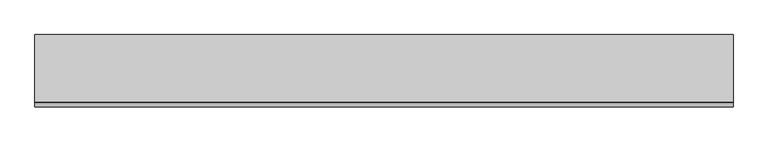
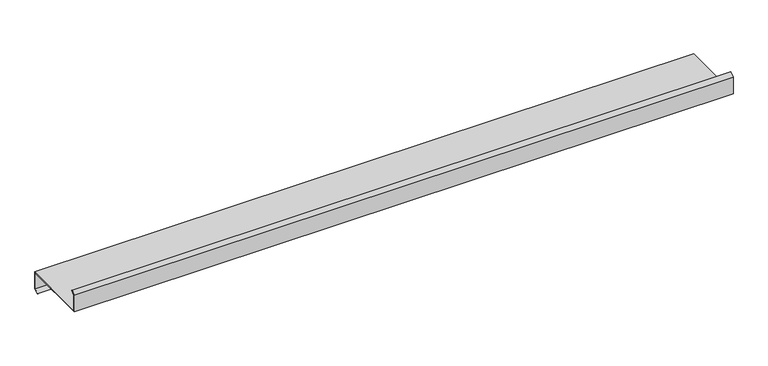
"""IFC4 building model written with IfcOpenShell, lengths in millimetres: proxy geometry, Generic Models 7:Generic Models 1:337419:Generic Models 1:337419 : Generic Models 7:Generic Models 1:337419:25 : Generic Models 7:Generic Models 1:337419:Generic Models 1:337419 : Generic Models 7:Generic Models 1:337419:301336."""

from ifc_helpers import new_model, si_unit, frame, origin, place, context, project, spatial, polyline, outline, extrude, source, transform, mapped, element, save


def generic_models_e2588900(model_context):
    return source(origin(), model_context, "Body", "SweptSolid", [
        extrude(outline(polyline([(-566667.6964303, 3711.7734375), (-566667.6964303, 3776.6625), (-566653.2894741, 3788.7513716), (-566651.3175393, 3786.7794368), (-566664.9183053, 3775.367039), (-566664.9183053, 3714.5515625), (-566413.6964303, 3714.5515625), (-566413.6964303, 3649.6625), (-566428.2895769, 3637.417396), (-566430.2615117, 3639.3893309), (-566416.4745553, 3650.957961), (-566416.4745553, 3711.7734375), (-566667.6964303, 3711.7734375)])), frame((599865.8367239, 0.0, 0.0), z_axis=(1.0, 0.0, 0.0), x_axis=(0.0, 1.0, 0.0)), (0.0, 0.0, 1.0), 2444.75),
    ])


if __name__ == "__main__":
    model = new_model("IFC4")
    model_context = context("Model", 3, world=origin())
    ifc_project = project(units=[si_unit("LENGTHUNIT", "METRE", prefix="MILLI")], contexts=[model_context])
    site = spatial("IfcSite", under=ifc_project)
    building = spatial("IfcBuilding", under=site)
    placement = place(None, origin())
    generic_models_shape = generic_models_e2588900(model_context)
    element("IfcBuildingElementProxy", 1, Name="Generic Models 7:Generic Models 1:337419:Generic Models 1:337419 : Generic Models 7:Generic Models 1:337419:25 : Generic Models 7:Generic Models 1:337419:Generic Models 1:337419 : Generic Models 7:Generic Models 1:337419:301336", ObjectType="Generic Models 7:Generic Models 1:337419:Generic Models 1:337419 : Generic Models 7:Generic Models 1:337419:25 : Generic Models 7:Generic Models 1:337419:Generic Models 1:337419 : Generic Models 7:Generic Models 1:337419:301336", at=placement, inside=building, context=model_context, shape_type="MappedRepresentation", body=[
        mapped(generic_models_shape, transform((0.0, 0.0, 0.0), x_axis=(1.0, 0.0, 0.0), y_axis=(0.0, 1.0, 0.0), z_axis=(0.0, 0.0, 1.0))),
    ])
    save(model, "model.ifc")

# Revit data of these elements
# Type "Generic Models 7:Generic Models 1:337419:Generic Models 1:337419 : Generic Models 7:Generic Models 1:337419:25 : Generic Models 7:Generic Models 1:337419:Generic Models 1:337419 : Generic Models 7:Generic Models 1:337419:301336"
#   NameOverride = "Generic Models 7:Generic Models 1:337419:Generic Models 1:337419 : Generic Models 7:Generic Models 1:337419:301336"
#   ObjectTypeOverride = "Generic Models 1:337419 : Generic Models 7:Generic Models 1:337419"
#   Reference = "Generic Models 1"
#   Tag = "301336"
# Element 1 (IfcBuildingElementProxy, "Generic Models 7:Generic Models 1:337419:Generic Models 1:337419 : Generic Models 7:Generic Models 1:337419:25 : Generic Models 7:Generic Models 1:337419:Generic Models 1:337419 : Generic Models 7:Generic Models 1:337419:301336")
#   Materials on its faces: "'ZEE' SECTION (8.0x3.5Z - SEE STRUCT. DWGS)"
# Materials
#   "'ZEE' SECTION (8.0x3.5Z - SEE STRUCT. DWGS)": class "Unassigned", colour RGB 210 209 208, transparency 0, Keynote = "M05121300.02", Cost = 0
